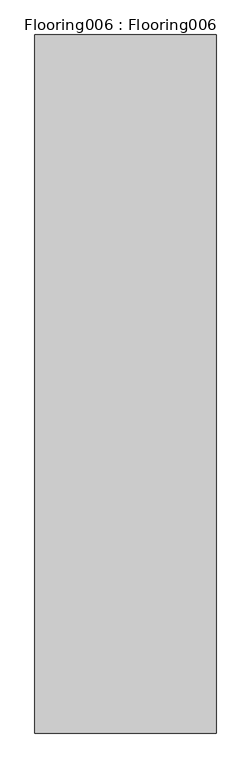
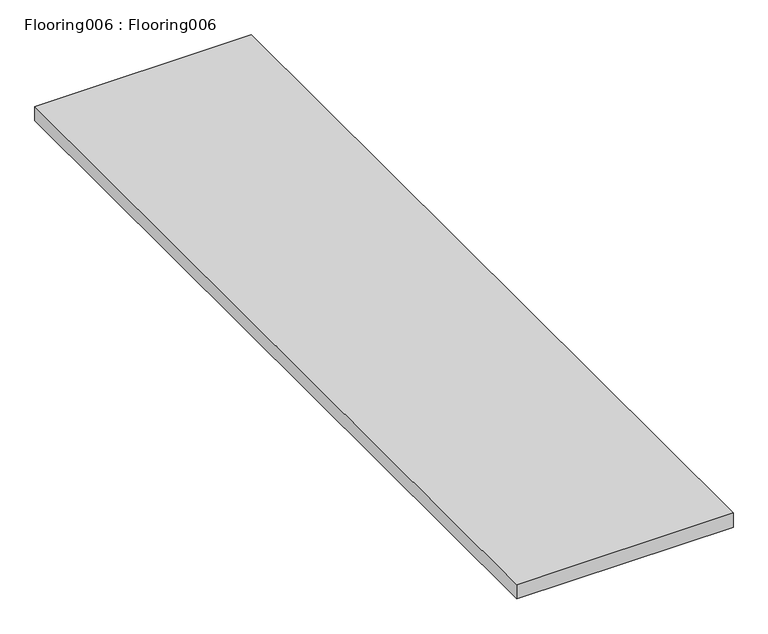
"""IFC4 building model written with IfcOpenShell, lengths in millimetres: proxy geometry, Flooring006 : Flooring006."""

from ifc_helpers import new_model, si_unit, frame, origin, place, context, project, spatial, polyline, outline, extrude, source, transform, mapped, element, save


def flooring006_flooring006_c1beb528(model_context):
    return source(origin(), model_context, "Body", "SweptSolid", [
        extrude(outline(polyline([(-5994.0708008, 7982.1531721), (-6513.0786133, 7982.1531721), (-6513.0786133, 9982.1531721), (-5994.0708008, 9982.1531721), (-5994.0708008, 7982.1531721)])), frame((0.0, 0.0, 40171.0155395), z_axis=(0.0, 0.0, 1.0), x_axis=(1.0, 0.0, 0.0)), (0.0, 0.0, 1.0), 35.7929688),
    ])


if __name__ == "__main__":
    model = new_model("IFC4")
    model_context = context("Model", 3, world=origin())
    ifc_project = project(units=[si_unit("LENGTHUNIT", "METRE", prefix="MILLI")], contexts=[model_context])
    site = spatial("IfcSite", under=ifc_project)
    building = spatial("IfcBuilding", under=site)
    placement = place(None, origin())
    flooring006_flooring006_shape = flooring006_flooring006_c1beb528(model_context)
    element("IfcBuildingElementProxy", 1, Name="Flooring006 : Flooring006", ObjectType="Flooring006 : Flooring006", at=placement, inside=building, context=model_context, shape_type="MappedRepresentation", body=[
        mapped(flooring006_flooring006_shape, transform((0.0, 0.0, 0.0), x_axis=(1.0, 0.0, 0.0), y_axis=(0.0, 1.0, 0.0), z_axis=(0.0, 0.0, 1.0))),
    ])
    save(model, "model.ifc")

# Revit data of these elements
# Type "Flooring006 : Flooring006"
#   NameOverride = "Flooring006"
# Element 1 (IfcBuildingElementProxy, "Flooring006 : Flooring006")
#   Materials on its faces: "TERRACE FLOORING TBD"
# Materials
#   "TERRACE FLOORING TBD": class "Unassigned", colour RGB 128 128 128, transparency 0
